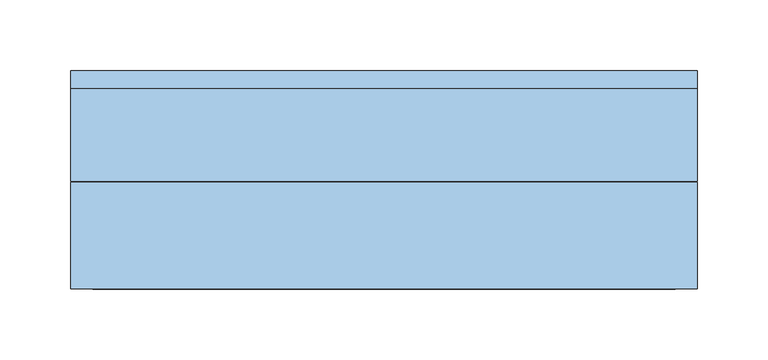
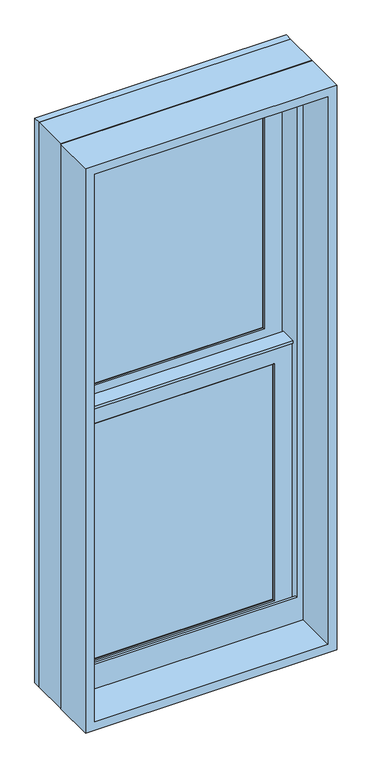
"""IFC4 building model written with IfcOpenShell, lengths in millimetres: window geometry, Window-Double_Hung-Marvin-Essential : ESDH1636."""

from ifc_helpers import new_model, si_unit, frame, origin, place, context, project, spatial, polyline, outline, extrude, faceted_brep, source, transform, mapped, element, save


def window_f56de130(model_context):
    return source(origin(), model_context, "Body", "SolidModel", [
        extrude(outline(polyline([(64.5583333, 20.6375), (64.5583333, 15.875), (45.5083333, 15.875), (45.5083333, 20.6375), (64.5583333, 20.6375)])), frame((0.0, 0.0, 1441.45), z_axis=(0.0, 0.0, 1.0), x_axis=(1.0, 0.0, 0.0)), (0.0, 0.0, 1.0), 450.85),
        extrude(outline(polyline([(-45.5083333, 20.6375), (-45.5083333, 15.875), (-64.5583333, 15.875), (-64.5583333, 20.6375), (-45.5083333, 20.6375)])), frame((0.0, 0.0, 1441.45), z_axis=(0.0, 0.0, 1.0), x_axis=(1.0, 0.0, 0.0)), (0.0, 0.0, 1.0), 450.85),
        extrude(outline(polyline([(165.1, 20.6375), (165.1, 15.875), (-165.1, 15.875), (-165.1, 20.6375), (165.1, 20.6375)])), frame((0.0, 0.0, 1657.35), z_axis=(0.0, 0.0, 1.0), x_axis=(1.0, 0.0, 0.0)), (0.0, 0.0, 1.0), 19.05),
        extrude(outline(polyline([(-64.5583333, 46.83125), (-64.5583333, 51.59375), (-45.5083333, 51.59375), (-45.5083333, 46.83125), (-64.5583333, 46.83125)])), frame((0.0, 0.0, 1930.4), z_axis=(0.0, 0.0, 1.0), x_axis=(1.0, 0.0, 0.0)), (0.0, 0.0, 1.0), 450.85),
        extrude(outline(polyline([(45.5083333, 46.83125), (45.5083333, 51.59375), (64.5583333, 51.59375), (64.5583333, 46.83125), (45.5083333, 46.83125)])), frame((0.0, 0.0, 1930.4), z_axis=(0.0, 0.0, 1.0), x_axis=(1.0, 0.0, 0.0)), (0.0, 0.0, 1.0), 450.85),
        extrude(outline(polyline([(-165.1, 46.83125), (-165.1, 51.59375), (165.1, 51.59375), (165.1, 46.83125), (-165.1, 46.83125)])), frame((0.0, 0.0, 2146.3), z_axis=(0.0, 0.0, 1.0), x_axis=(1.0, 0.0, 0.0)), (0.0, 0.0, 1.0), 19.05),
        extrude(outline(polyline([(64.5583333, 20.6375), (45.5083333, 20.6375), (45.5083333, 25.4), (64.5583333, 25.4), (64.5583333, 20.6375)])), frame((0.0, 0.0, 1441.45), z_axis=(0.0, 0.0, 1.0), x_axis=(1.0, 0.0, 0.0)), (0.0, 0.0, 1.0), 450.85),
        extrude(outline(polyline([(-45.5083333, 20.6375), (-64.5583333, 20.6375), (-64.5583333, 25.4), (-45.5083333, 25.4), (-45.5083333, 20.6375)])), frame((0.0, 0.0, 1441.45), z_axis=(0.0, 0.0, 1.0), x_axis=(1.0, 0.0, 0.0)), (0.0, 0.0, 1.0), 450.85),
        extrude(outline(polyline([(165.1, 20.6375), (-165.1, 20.6375), (-165.1, 25.4), (165.1, 25.4), (165.1, 20.6375)])), frame((0.0, 0.0, 1657.35), z_axis=(0.0, 0.0, 1.0), x_axis=(1.0, 0.0, 0.0)), (0.0, 0.0, 1.0), 19.05),
        extrude(outline(polyline([(-64.5583333, 56.35625), (-45.5083333, 56.35625), (-45.5083333, 51.59375), (-64.5583333, 51.59375), (-64.5583333, 56.35625)])), frame((0.0, 0.0, 1930.4), z_axis=(0.0, 0.0, 1.0), x_axis=(1.0, 0.0, 0.0)), (0.0, 0.0, 1.0), 450.85),
        extrude(outline(polyline([(45.5083333, 56.35625), (64.5583333, 56.35625), (64.5583333, 51.59375), (45.5083333, 51.59375), (45.5083333, 56.35625)])), frame((0.0, 0.0, 1930.4), z_axis=(0.0, 0.0, 1.0), x_axis=(1.0, 0.0, 0.0)), (0.0, 0.0, 1.0), 450.85),
        extrude(outline(polyline([(-165.1, 56.35625), (165.1, 56.35625), (165.1, 51.59375), (-165.1, 51.59375), (-165.1, 56.35625)])), frame((0.0, 0.0, 2146.3), z_axis=(0.0, 0.0, 1.0), x_axis=(1.0, 0.0, 0.0)), (0.0, 0.0, 1.0), 19.05),
        faceted_brep([(-192.0875, 5.6780605, 1922.3351748), (-192.0875, 5.6780605, 1917.7), (192.0875, 5.6780605, 1917.7), (192.0875, 5.6780605, 1922.3351748), (-192.0875, 34.8118605, 1922.3351748), (192.0875, 34.8118605, 1922.3351748), (192.0875, 34.8118605, 1917.7), (-192.0875, 34.8118605, 1917.7), (-192.0875, 30.1625, 1917.7), (-192.0875, 30.1625, 1414.4625), (-192.0875, 8.9241104, 1414.4625), (-192.0875, 8.9241104, 1917.7), (192.0875, 8.9241104, 1917.7), (192.0875, 30.1625, 1917.7), (192.0875, 8.9241104, 1414.4625), (192.0875, 30.1625, 1414.4625), (-176.2034752, 11.90625, 1903.4034752), (-176.2034752, 30.1625, 1903.4034752), (176.2034752, 30.1625, 1903.4034752), (176.2034752, 11.90625, 1903.4034752), (-159.54375, 10.4662439, 1886.74375), (-159.54375, 11.90625, 1886.74375), (159.54375, 11.90625, 1886.74375), (159.54375, 10.4662439, 1886.74375), (161.0858834, 8.9241104, 1888.2858834), (-161.0858834, 8.9241104, 1888.2858834), (176.2034752, 30.1625, 1430.3465248), (176.2034752, 11.90625, 1430.3465248), (159.54375, 11.90625, 1447.00625), (159.54375, 10.4662439, 1447.00625), (161.0858834, 8.9241104, 1445.4641166), (-176.2034752, 30.1625, 1430.3465248), (-176.2034752, 11.90625, 1430.3465248), (-159.54375, 11.90625, 1447.00625), (-159.54375, 10.4662439, 1447.00625), (-161.0858834, 8.9241104, 1445.4641166)], [[[0, 1, 2, 3]], [[4, 5, 6, 7]], [[1, 0, 4, 7, 8, 9, 10, 11]], [[2, 1, 11, 12]], [[7, 6, 13, 8]], [[3, 2, 12, 14, 15, 13, 6, 5]], [[0, 3, 5, 4]], [[16, 17, 18, 19]], [[20, 21, 22, 23]], [[20, 23, 24, 25]], [[19, 18, 26, 27]], [[23, 22, 28, 29]], [[24, 23, 29, 30]], [[27, 26, 31, 32]], [[29, 28, 33, 34]], [[30, 29, 34, 35]], [[15, 14, 10, 9]], [[15, 9, 8, 13], [18, 17, 31, 26]], [[17, 16, 32, 31]], [[16, 19, 27, 32], [22, 21, 33, 28]], [[21, 20, 34, 33]], [[20, 25, 35, 34]], [[10, 14, 12, 11], [25, 24, 30, 35]]]),
        extrude(outline(polyline([(38.5955581, 1903.4125), (33.5778968, 1903.4125), (33.5778968, 1905.0), (39.9405976, 1905.0), (39.9405976, 1903.4125), (61.515625, 1903.4125), (47.6307501, 1900.0975159), (38.5955581, 1900.0975159), (38.5955581, 1903.4125)])), frame((-192.0875, 0.0, 0.0), z_axis=(1.0, 0.0, 0.0), x_axis=(0.0, 1.0, 0.0)), (0.0, 0.0, 1.0), 384.175),
        faceted_brep([(222.25, 0.0, 1384.3), (222.25, 0.0, 2438.4), (-222.25, 0.0, 2438.4), (-222.25, 0.0, 1384.3), (196.05625, 0.0, 1445.41875), (-196.05625, 0.0, 1445.41875), (-196.05625, 0.0, 2412.20625), (196.05625, 0.0, 2412.20625), (196.05625, 3.96875, 1384.3), (-196.05625, 3.96875, 1384.3), (-196.05625, 3.96875, 1445.41875), (196.05625, 3.96875, 1445.41875), (-222.25, 65.6828125, 1384.3), (-196.05625, 65.6828125, 1384.3), (196.05625, 65.6828125, 1384.3), (222.25, 65.6828125, 1384.3), (-222.25, 65.6828125, 2438.4), (222.25, 65.6828125, 2438.4), (196.05625, 65.6828125, 2412.20625), (-196.05625, 65.6828125, 2412.20625)], [[[0, 1, 2, 3], [4, 5, 6, 7]], [[8, 9, 10, 11]], [[5, 4, 11, 10]], [[0, 3, 12, 13, 9, 8, 14, 15]], [[13, 12, 16, 17, 15, 14, 18, 19]], [[13, 19, 6, 5, 10, 9]], [[7, 6, 19, 18]], [[18, 14, 8, 11, 4, 7]], [[1, 0, 15, 17]], [[2, 1, 17, 16]], [[3, 2, 16, 12]]]),
        faceted_brep([(196.05625, 30.1625, 1911.35), (194.46875, 30.1625, 1911.35), (194.46875, 30.1625, 1408.6544613), (196.05625, 30.1625, 1408.6544613), (-194.46875, 30.1625, 1911.35), (-196.05625, 30.1625, 1911.35), (-196.05625, 30.1625, 1408.6544613), (-194.46875, 30.1625, 1408.6544613), (194.46875, 63.5, 1911.35), (196.05625, 63.5, 1911.35), (196.05625, 63.5, 1402.1743077), (194.46875, 63.5, 1402.1743077), (-196.05625, 63.5, 1911.35), (-194.46875, 63.5, 1911.35), (-194.46875, 63.5, 1402.1743077), (-196.05625, 63.5, 1402.1743077), (207.3108932, 3.96875, 1413.7460105), (207.3108932, 3.96875, 1384.3), (207.3108932, 65.6828125, 1384.3), (207.3108932, 65.6828125, 1401.750012), (-207.3108932, 3.96875, 1384.3), (-207.3108932, 3.96875, 1413.7460105), (-207.3108932, 65.6828125, 1401.750012), (-207.3108932, 65.6828125, 1384.3), (207.3108932, 78.58125, 1399.2428097), (-207.3108932, 78.58125, 1399.2428097), (-205.2971252, 68.2348864, 1401.2539391), (-187.33135, 68.2348864, 1401.2539391), (-187.33135, 65.6828125, 1401.750012), (187.33135, 65.6828125, 1401.750012), (187.33135, 68.2348864, 1401.2539391), (205.2971252, 68.2348864, 1401.2539391), (-222.25, 65.6828125, 1384.3), (-222.25, 78.5948249, 1384.3), (222.25, 78.5948249, 1384.3), (222.25, 65.6828125, 1384.3), (-222.25, 78.58125, 2438.4), (222.25, 78.58125, 2438.4), (207.3108932, 78.58125, 2423.4608932), (-207.3108932, 78.58125, 2423.4608932), (-222.25, 65.6828125, 2438.4), (-205.2971252, 68.2348864, 2421.4471252), (205.2971252, 68.2348864, 2421.4471252), (187.33135, 68.2348864, 2403.48135), (-187.33135, 68.2348864, 2403.48135), (-187.33135, 65.6828125, 2403.48135), (187.33135, 65.6828125, 2403.48135), (222.25, 65.6828125, 2438.4)], [[[0, 1, 2, 3]], [[4, 5, 6, 7]], [[8, 9, 10, 11]], [[12, 13, 14, 15]], [[1, 8, 11, 2]], [[9, 0, 3, 10]], [[1, 0, 9, 8]], [[5, 4, 13, 12]], [[5, 12, 15, 6]], [[13, 4, 7, 14]], [[16, 17, 18, 19]], [[20, 21, 22, 23]], [[24, 25, 26, 27, 28, 22, 21, 16, 19, 29, 30, 31], [3, 2, 11, 10], [7, 6, 15, 14]], [[17, 16, 21, 20]], [[17, 20, 23, 32, 33, 34, 35, 18]], [[34, 33, 36, 37], [25, 24, 38, 39]], [[33, 32, 40, 36]], [[39, 41, 26, 25]], [[41, 42, 31, 30, 43, 44, 27, 26]], [[44, 45, 28, 27]], [[40, 32, 23, 22, 28, 45, 46, 29, 19, 18, 35, 47]], [[36, 40, 47, 37]], [[39, 38, 42, 41]], [[44, 43, 46, 45]], [[34, 37, 47, 35]], [[42, 38, 24, 31]], [[46, 43, 30, 29]]]),
        extrude(outline(polyline([(172.24375, 11.90625), (-172.24375, 11.90625), (-172.24375, 15.08125), (172.24375, 15.08125), (172.24375, 11.90625)])), frame((0.0, 0.0, 1434.30625), z_axis=(0.0, 0.0, 1.0), x_axis=(1.0, 0.0, 0.0)), (0.0, 0.0, 1.0), 465.1375),
        extrude(outline(polyline([(172.24375, 42.8625), (-172.24375, 42.8625), (-172.24375, 46.0375), (172.24375, 46.0375), (172.24375, 42.8625)])), frame((0.0, 0.0, 1923.25625), z_axis=(0.0, 0.0, 1.0), x_axis=(1.0, 0.0, 0.0)), (0.0, 0.0, 1.0), 465.1375),
        faceted_brep([(-159.54375, 31.194477, 1886.74375), (-161.0858834, 32.7366104, 1888.2858834), (161.0858834, 32.7366104, 1888.2858834), (159.54375, 31.194477, 1886.74375), (-159.54375, 30.1625, 1886.74375), (159.54375, 30.1625, 1886.74375), (-192.0875, 32.7366104, 1919.2875), (-192.0875, 30.1625, 1919.2875), (192.0875, 30.1625, 1919.2875), (192.0875, 32.7366104, 1919.2875), (161.0858834, 32.7366104, 1445.4641166), (159.54375, 31.194477, 1447.00625), (159.54375, 30.1625, 1447.00625), (192.0875, 30.1625, 1414.4625), (192.0875, 32.7366104, 1414.4625), (-161.0858834, 32.7366104, 1445.4641166), (-159.54375, 31.194477, 1447.00625), (-159.54375, 30.1625, 1447.00625), (-192.0875, 30.1625, 1414.4625), (-192.0875, 32.7366104, 1414.4625)], [[[0, 1, 2, 3]], [[4, 0, 3, 5]], [[6, 7, 8, 9]], [[3, 2, 10, 11]], [[5, 3, 11, 12]], [[9, 8, 13, 14]], [[11, 10, 15, 16]], [[12, 11, 16, 17]], [[14, 13, 18, 19]], [[9, 14, 19, 6], [1, 15, 10, 2]], [[16, 15, 1, 0]], [[17, 16, 0, 4]], [[7, 18, 13, 8], [5, 12, 17, 4]], [[19, 18, 7, 6]]]),
        faceted_brep([(-176.2034752, 42.8625, 2392.3534752), (-176.2034752, 61.11875, 2392.3534752), (176.2034752, 61.11875, 2392.3534752), (176.2034752, 42.8625, 2392.3534752), (-159.54375, 41.4224939, 2375.69375), (-159.54375, 42.8625, 2375.69375), (159.54375, 42.8625, 2375.69375), (159.54375, 41.4224939, 2375.69375), (-161.0858834, 39.8803604, 2377.2358834), (161.0858834, 39.8803604, 2377.2358834), (-192.0875, 61.11875, 2408.2375), (-192.0875, 39.8803604, 2408.2375), (192.0875, 39.8803604, 2408.2375), (192.0875, 61.11875, 2408.2375), (176.2034752, 61.11875, 1919.2965248), (176.2034752, 42.8625, 1919.2965248), (159.54375, 42.8625, 1935.95625), (159.54375, 41.4224939, 1935.95625), (161.0858834, 39.8803604, 1934.4141166), (192.0875, 39.8803604, 1903.4125), (192.0875, 61.11875, 1903.4125), (-176.2034752, 61.11875, 1919.2965248), (-176.2034752, 42.8625, 1919.2965248), (-159.54375, 42.8625, 1935.95625), (-159.54375, 41.4224939, 1935.95625), (-161.0858834, 39.8803604, 1934.4141166), (-192.0875, 39.8803604, 1903.4125), (-192.0875, 61.11875, 1903.4125)], [[[0, 1, 2, 3]], [[4, 5, 6, 7]], [[8, 4, 7, 9]], [[10, 11, 12, 13]], [[3, 2, 14, 15]], [[7, 6, 16, 17]], [[9, 7, 17, 18]], [[13, 12, 19, 20]], [[15, 14, 21, 22]], [[17, 16, 23, 24]], [[18, 17, 24, 25]], [[20, 19, 26, 27]], [[13, 20, 27, 10], [1, 21, 14, 2]], [[22, 21, 1, 0]], [[3, 15, 22, 0], [5, 23, 16, 6]], [[24, 23, 5, 4]], [[25, 24, 4, 8]], [[11, 26, 19, 12], [9, 18, 25, 8]], [[27, 26, 11, 10]]]),
        faceted_brep([(-192.0875, 61.11875, 1903.4125), (-192.0875, 63.6928604, 1903.4125), (192.0875, 63.6928604, 1903.4125), (192.0875, 61.11875, 1903.4125), (-159.54375, 62.150727, 1935.95625), (-159.54375, 61.11875, 1935.95625), (159.54375, 61.11875, 1935.95625), (159.54375, 62.150727, 1935.95625), (-161.0858834, 63.6928604, 1934.4141166), (161.0858834, 63.6928604, 1934.4141166), (192.0875, 63.6928604, 2408.2375), (192.0875, 61.11875, 2408.2375), (159.54375, 61.11875, 2375.69375), (159.54375, 62.150727, 2375.69375), (161.0858834, 63.6928604, 2377.2358834), (-192.0875, 63.6928604, 2408.2375), (-192.0875, 61.11875, 2408.2375), (-159.54375, 61.11875, 2375.69375), (-159.54375, 62.150727, 2375.69375), (-161.0858834, 63.6928604, 2377.2358834)], [[[0, 1, 2, 3]], [[4, 5, 6, 7]], [[8, 4, 7, 9]], [[3, 2, 10, 11]], [[7, 6, 12, 13]], [[9, 7, 13, 14]], [[11, 10, 15, 16]], [[13, 12, 17, 18]], [[14, 13, 18, 19]], [[16, 15, 1, 0]], [[3, 11, 16, 0], [5, 17, 12, 6]], [[18, 17, 5, 4]], [[19, 18, 4, 8]], [[1, 15, 10, 2], [9, 14, 19, 8]]]),
        extrude(outline(polyline([(172.24375, 26.19375), (-172.24375, 26.19375), (-172.24375, 30.1625), (172.24375, 30.1625), (172.24375, 26.19375)])), frame((0.0, 0.0, 1434.30625), z_axis=(0.0, 0.0, 1.0), x_axis=(1.0, 0.0, 0.0)), (0.0, 0.0, 1.0), 465.1375),
        extrude(outline(polyline([(172.24375, 57.15), (-172.24375, 57.15), (-172.24375, 61.11875), (172.24375, 61.11875), (172.24375, 57.15)])), frame((0.0, 0.0, 1923.25625), z_axis=(0.0, 0.0, 1.0), x_axis=(1.0, 0.0, 0.0)), (0.0, 0.0, 1.0), 465.1375),
        extrude(outline(polyline([(2438.4, 222.25), (2438.4, -222.25), (1384.3, -222.25), (1384.3, 222.25), (2438.4, 222.25)]), holes=[polyline([(2422.525, 206.375), (1400.175, 206.375), (1400.175, -206.375), (2422.525, -206.375), (2422.525, 206.375)])]), frame((0.0, -76.2, 0.0), z_axis=(0.0, 1.0, 0.0), x_axis=(0.0, 0.0, 1.0)), (0.0, 0.0, 1.0), 75.40625),
    ])


if __name__ == "__main__":
    model = new_model("IFC4")
    model_context = context("Model", 3, world=origin())
    ifc_project = project(units=[si_unit("LENGTHUNIT", "METRE", prefix="MILLI")], contexts=[model_context])
    site = spatial("IfcSite", under=ifc_project)
    building = spatial("IfcBuilding", under=site)
    placement = place(None, origin())
    window_shape = window_f56de130(model_context)
    element("IfcWindow", 1, ObjectType="Window-Double_Hung-Marvin-Essential : ESDH1636", at=placement, inside=building, context=model_context, shape_type="MappedRepresentation", body=[
        mapped(window_shape, transform((0.0, 0.0, 0.0), x_axis=(1.0, 0.0, 0.0), y_axis=(0.0, 1.0, 0.0), z_axis=(0.0, 0.0, 1.0))),
    ])
    save(model, "model.ifc")

# Revit data of these elements
# Type "Window-Double_Hung-Marvin-Essential : ESDH1636"
#   Type Mark = "40"
#   Window Type = "Essential Double Hung"
#   Product data url = "https://bimobject.com/marvin-windows-and-doors/product/marvin-dhwau"
#   Product Guid = "c4a96547-874c-4385-91dc-a058adc19d98"
#   Frame = "All Ultrex"
#   Egress Window = "No"
#   URL = "www.marvin.com"
#   Model = "ESDH1636"
#   Manufacturer = "Marvin Windows and Doors"
#   Label Egress = ""
#   Glass Type = "IG Low E II with Argon"
#   Design Pressure = "DP50"
#   Description = "1842 DBHG"
#   Analytic Construction = "<None>"
#   Prairie Corner Width = 0' - 4"
#   Prairie Corner Height = 0' - 4"
#   Egress Width = 1' - 2 9/16"
#   Egress Height = 1' - 4 27/128"
#   Rough Width = 1' - 6"
#   Rough Height = 3' - 6"
#   Nominal Width = 1' - 6"
#   Nominal Height = 3' - 6"
#   Inset to Installation Flange [instance default] = 0' - 1"
#   Height = 3' - 5 1/2"
#   Egress Area = 1.63939 SF
#   Default Head Height = 8' - 0"
#   Width = 1' - 5 1/2"
#   Daylight Area = 3.02067 SF
#   DLO Width = 1' - 0 9/16"
#   DLO Height = 1' - 5 5/16"
#   Muntins Top Sash = yes
#   Lites Wide Top Sash = 3
#   Lites Wide Bottom Sash = 3
#   Lites High Top Sash = 2
#   Lites High Bottom Sash = 2
#   Lite Cut Prairie 9 = no
#   Lite Cut HV Grid = yes
#   Muntins Bottom Sash = yes
#   Label Visibility = no
#   Jamb Extension Visibility = yes
#   Edition number = 1
#   Interior Material = Ultrex-Marvin-Stonewhite
#   Glazing Material = Glass-Marvin-IG Low E II with Argon
#   Cladding Material = Ultrex-Marvin-Pebblegray
#   Wall Closure = (empty or 0)
#   Assembly Code = ""
# Element 1 (IfcWindow, "Window-Double_Hung-Marvin-Essential : ESDH1636")
#   Materials on its faces: "Ultrex-Marvin-Pebblegray", "Ultrex-Marvin-Stonewhite", "Glass-Marvin-IG Low E II with Argon"
# Materials
#   "Ultrex-Marvin-Stonewhite": class "Paint", colour RGB 250 251 245, transparency 0
#   "Glass-Marvin-IG Low E II with Argon": class "Glass", colour RGB 0 128 192, transparency 0.85
#   "Ultrex-Marvin-Pebblegray": class "Paint", colour RGB 189 185 173, transparency 0
